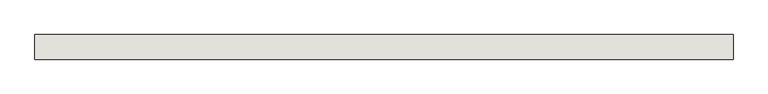
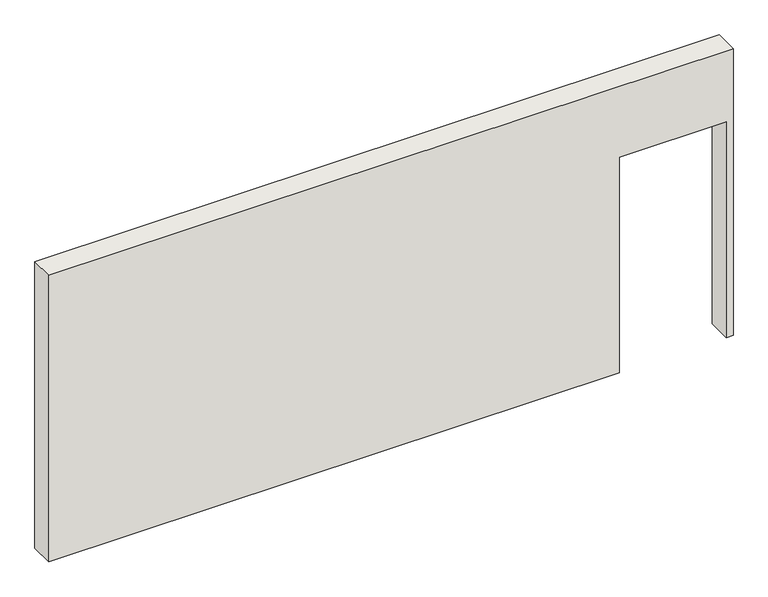
"""IFC4 building model written with IfcOpenShell, lengths in millimetres: wall geometry, Holzwand."""

from ifc_helpers import new_model, si_unit, frame, origin, place, context, project, spatial, polyline, outline, extrude, source, transform, mapped, element, save


def wall_c528e420(model_context):
    return source(origin(), model_context, "Body", "SweptSolid", [
        extrude(outline(polyline([(0.0, 4727.1048224), (1890.0, 4727.1048224), (1890.0, 5612.1048224), (0.0, 5612.1048224), (0.0, 5670.0), (2510.0, 5670.0), (2510.0, 0.0), (0.0, 0.0), (0.0, 4727.1048224)])), frame((0.0, 0.0, 0.0), z_axis=(0.0, 1.0, 0.0), x_axis=(0.0, 0.0, 1.0)), (0.0, 0.0, 1.0), 200.0),
    ])


if __name__ == "__main__":
    model = new_model("IFC4")
    model_context = context("Model", 3, world=origin())
    ifc_project = project(units=[si_unit("LENGTHUNIT", "METRE", prefix="MILLI")], contexts=[model_context])
    site = spatial("IfcSite", under=ifc_project)
    building = spatial("IfcBuilding", under=site)
    placement = place(None, origin())
    wall_shape = wall_c528e420(model_context)
    element("IfcWall", 1, ObjectType="Holzwand", at=placement, inside=building, context=model_context, shape_type="MappedRepresentation", body=[
        mapped(wall_shape, transform((0.0, 0.0, 0.0), x_axis=(1.0, 0.0, 0.0), y_axis=(0.0, 1.0, 0.0), z_axis=(0.0, 0.0, 1.0))),
    ])
    save(model, "model.ifc")

# Revit data of these elements
# Element 1 (IfcWall, "Holzwand")
#   Materials on its faces: "holzschalung"
# Materials
#   "holzschalung": class "Unassigned", colour RGB 128 128 128, transparency 0
